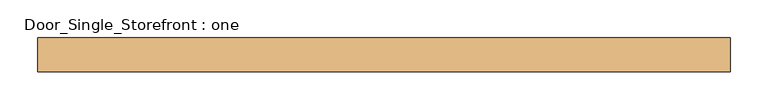
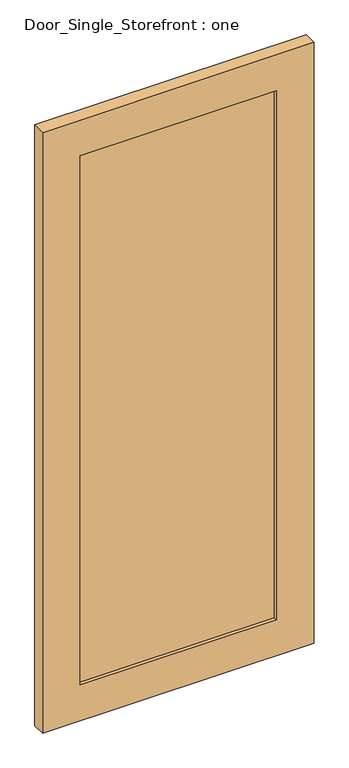
"""IFC4 building model written with IfcOpenShell, lengths in millimetres: door geometry, Door_Single_Storefront : one."""

from ifc_helpers import new_model, si_unit, frame, origin, place, context, project, spatial, polyline, outline, extrude, source, transform, mapped, element, save


def door_single_storefront_one_0dbe0f4e(model_context):
    return source(origin(), model_context, "Body", "SweptSolid", [
        extrude(outline(polyline([(330.2, 6.35), (330.2, -12.7), (-330.2, -12.7), (-330.2, 6.35), (330.2, 6.35)])), frame((0.0, 0.0, 127.0), z_axis=(0.0, 0.0, 1.0), x_axis=(1.0, 0.0, 0.0)), (0.0, 0.0, 1.0), 1881.1875),
        extrude(outline(polyline([(2135.1875, -457.2), (0.0, -457.2), (0.0, 457.2), (2135.1875, 457.2), (2135.1875, -457.2)]), holes=[polyline([(127.0, 330.2), (127.0, -330.2), (2008.1875, -330.2), (2008.1875, 330.2), (127.0, 330.2)])]), frame((0.0, -25.4, 0.0), z_axis=(0.0, 1.0, 0.0), x_axis=(0.0, 0.0, 1.0)), (0.0, 0.0, 1.0), 44.45),
    ])


if __name__ == "__main__":
    model = new_model("IFC4")
    model_context = context("Model", 3, world=origin())
    ifc_project = project(units=[si_unit("LENGTHUNIT", "METRE", prefix="MILLI")], contexts=[model_context])
    site = spatial("IfcSite", under=ifc_project)
    building = spatial("IfcBuilding", under=site)
    placement = place(None, origin())
    door_single_storefront_one_shape = door_single_storefront_one_0dbe0f4e(model_context)
    element("IfcDoor", 1, ObjectType="Door_Single_Storefront : one", at=placement, inside=building, context=model_context, shape_type="MappedRepresentation", body=[
        mapped(door_single_storefront_one_shape, transform((0.0, 0.0, 0.0), x_axis=(1.0, 0.0, 0.0), y_axis=(0.0, 1.0, 0.0), z_axis=(0.0, 0.0, 1.0))),
    ])
    save(model, "model.ifc")

# Revit data of these elements
# Type "Door_Single_Storefront : one"
#   Type Mark = "29"
#   Analytic Construction = "<None>"
#   Stile_Width = 0' - 5"
#   Door_Thickness = 0' - 1 3/4"
#   Door_Offset = 0' - 1"
#   Glass_Material = ALUM. STOREFRONT W/ INSULATED GLAZING
#   Frame_Material = Aluminum
#   Function = (empty or 0)
# Element 1 (IfcDoor, "Door_Single_Storefront : one")
#   Materials on its faces: "Aluminum", "ALUM. STOREFRONT W/ INSULATED GLAZING"
# Materials
#   "ALUM. STOREFRONT W/ INSULATED GLAZING": class "Glass", colour RGB 196 205 210, transparency 0.85, Description = "Soda Lime Glass", Cost = 0
#   "Aluminum": class "Metal", colour RGB 244 244 244, transparency 0, Description = "Aluminum 6061", Cost = 0
